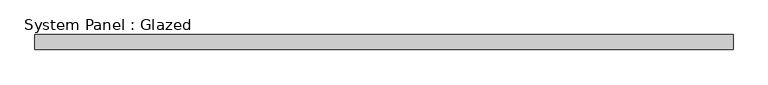
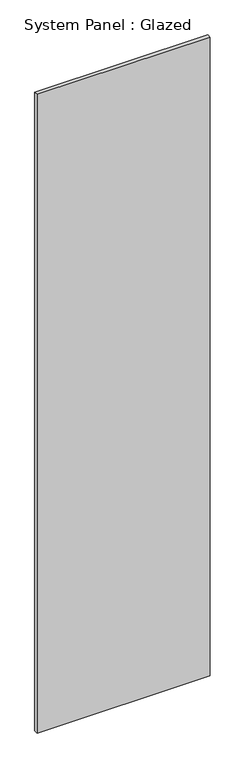
"""IFC4 building model written with IfcOpenShell, lengths in millimetres: plate geometry, System Panel : Glazed."""

import ifcopenshell
import ifcopenshell.guid

model = None  # the IFC model being written
_history = None  # IfcOwnerHistory: only IFC2X3 demands one
_inside = {}  # id of a spatial element -> (the spatial element, [elements in it])
_under = {}  # id of a project, library or spatial element -> (it, [spatial elements below it])
_declared = {}  # id of a project -> (the project, [libraries it declares])
_typed = {}  # id of a type object -> (the type object, [elements of that type])
_made_of = {}  # id of a material, layer set ... -> (it, [elements and type objects made of it])


def new_model(schema):
    """Start an empty IFC model of exactly this schema.

    Asked for "IFC4X3", IfcOpenShell would pick the latest addendum, in which some entities
    have other attributes; the version numbers below select the first issue.
    IFC2X3 requires an IfcOwnerHistory on every rooted entity: one is made here for all.
    """
    global model, _history
    if schema == "IFC4X3":
        model = ifcopenshell.file(schema_version=(4, 3, 0, 0))
    else:
        model = ifcopenshell.file(schema=schema)
    _inside.clear()
    _under.clear()
    _declared.clear()
    _typed.clear()
    _made_of.clear()
    _history = None
    if model.schema == "IFC2X3":
        org = make("IfcOrganization", Name="unknown")
        user = make(
            "IfcPersonAndOrganization",
            ThePerson=make("IfcPerson", FamilyName="unknown"),
            TheOrganization=org,
        )
        app = make(
            "IfcApplication",
            ApplicationDeveloper=org,
            Version="unknown",
            ApplicationFullName="unknown",
            ApplicationIdentifier="unknown",
        )
        _history = make(
            "IfcOwnerHistory",
            OwningUser=user,
            OwningApplication=app,
            ChangeAction="ADDED",
            CreationDate=0,
        )
    return model


def make(cls, **values):
    """One entity of the class cls with the attributes given. An attribute that is None is left unset."""
    return model.create_entity(
        cls, **{name: value for name, value in values.items() if value is not None}
    )


def rooted(cls, **values):
    """An entity with a GlobalId (a new one), such as an element, a storey or a relation."""
    return make(cls, GlobalId=ifcopenshell.guid.new(), OwnerHistory=_history, **values)


def si_unit(unit_type, name, prefix=None):
    """IfcSIUnit, for example si_unit("LENGTHUNIT", "METRE", prefix="MILLI")."""
    return make("IfcSIUnit", UnitType=unit_type, Prefix=prefix, Name=name)


def assignment(units):
    """IfcUnitAssignment: the units of a project."""
    return None if units is None else make("IfcUnitAssignment", Units=units)


def point(xyz):
    """IfcCartesianPoint."""
    return None if xyz is None else make("IfcCartesianPoint", Coordinates=xyz)


def direction(xyz):
    """IfcDirection."""
    return None if xyz is None else make("IfcDirection", DirectionRatios=xyz)


def frame(location, z_axis=None, x_axis=None):
    """IfcAxis2Placement3D, a coordinate frame: its origin and axes. An axis left out is left unset."""
    return make(
        "IfcAxis2Placement3D",
        Location=point(location),
        Axis=direction(z_axis),
        RefDirection=direction(x_axis),
    )


def origin():
    """The frame at (0, 0, 0) with its axes left unset."""
    return frame((0.0, 0.0, 0.0))


def origin_with_axes():
    """The frame at (0, 0, 0) with the z axis (0, 0, 1) and the x axis (1, 0, 0) written out."""
    return frame((0.0, 0.0, 0.0), z_axis=(0.0, 0.0, 1.0), x_axis=(1.0, 0.0, 0.0))


def place(relative_to, where):
    """IfcLocalPlacement: puts the frame where relative to a parent placement (None: the world)."""
    return make(
        "IfcLocalPlacement", PlacementRelTo=relative_to, RelativePlacement=where
    )


def context(
    kind, dimensions, precision=None, world=None, true_north=None, identifier=None
):
    """IfcGeometricRepresentationContext, for example the 3D "Model" context."""
    return make(
        "IfcGeometricRepresentationContext",
        ContextIdentifier=identifier,
        ContextType=kind,
        CoordinateSpaceDimension=dimensions,
        Precision=precision,
        WorldCoordinateSystem=world,
        TrueNorth=true_north,
    )


def project(units=None, contexts=None):
    """IfcProject with its units and contexts."""
    return rooted(
        "IfcProject",
        Name="project",
        RepresentationContexts=contexts,
        UnitsInContext=assignment(units),
    )


def spatial(cls, under=None, at=None, **own):
    """A site, building, storey or space (cls), placed at a placement, below another one or the project."""
    s = rooted(cls, ObjectPlacement=at, **own)
    if under is not None:
        _under.setdefault(under.id(), (under, []))[1].append(s)
    return s


def polyline(points):
    """IfcPolyline through the points."""
    return make("IfcPolyline", Points=[point(p) for p in points])


def outline(outer, holes=None, kind="AREA"):
    """IfcArbitraryClosedProfileDef: a profile drawn as a closed curve; with holes, ...WithVoids."""
    if holes is None:
        return make("IfcArbitraryClosedProfileDef", ProfileType=kind, OuterCurve=outer)
    return make(
        "IfcArbitraryProfileDefWithVoids",
        ProfileType=kind,
        OuterCurve=outer,
        InnerCurves=holes,
    )


def extrude(swept, where, along, depth):
    """IfcExtrudedAreaSolid: the profile swept, set in the frame where, extruded along a direction by depth."""
    return make(
        "IfcExtrudedAreaSolid",
        SweptArea=swept,
        Position=where,
        ExtrudedDirection=direction(along),
        Depth=depth,
    )


def shape(context_of_items, identifier, shape_type, items):
    """IfcShapeRepresentation: the items that make up one representation, for example the "Body"."""
    return make(
        "IfcShapeRepresentation",
        ContextOfItems=context_of_items,
        RepresentationIdentifier=identifier,
        RepresentationType=shape_type,
        Items=items,
    )


def source(mapping_origin, context_of_items, identifier, shape_type, items):
    """IfcRepresentationMap: a shape defined once, which mapped items show again and again."""
    return make(
        "IfcRepresentationMap",
        MappingOrigin=mapping_origin,
        MappedRepresentation=shape(context_of_items, identifier, shape_type, items),
    )


def transform(
    local_origin,
    x_axis=None,
    y_axis=None,
    z_axis=None,
    scale=None,
    scale2=None,
    scale3=None,
    uniform=True,
):
    """IfcCartesianTransformationOperator3D, or its non-uniform kind. x_axis, y_axis, z_axis: its Axis1, 2, 3."""
    if uniform:
        return make(
            "IfcCartesianTransformationOperator3D",
            Axis1=direction(x_axis),
            Axis2=direction(y_axis),
            LocalOrigin=point(local_origin),
            Scale=scale,
            Axis3=direction(z_axis),
        )
    return make(
        "IfcCartesianTransformationOperator3DnonUniform",
        Axis1=direction(x_axis),
        Axis2=direction(y_axis),
        LocalOrigin=point(local_origin),
        Scale=scale,
        Axis3=direction(z_axis),
        Scale2=scale2,
        Scale3=scale3,
    )


def mapped(mapping_source, mapping_target):
    """IfcMappedItem: shows the shape of a source again, moved by a transform."""
    return make(
        "IfcMappedItem", MappingSource=mapping_source, MappingTarget=mapping_target
    )


def made_of(thing, what):
    """Note that an element or type object is made of a material, layer set ...; save() writes the relation."""
    if what is not None:
        _made_of.setdefault(what.id(), (what, []))[1].append(thing)
    return thing


def element(
    cls,
    number,
    at=None,
    inside=None,
    cuts=None,
    type_object=None,
    material=None,
    context=None,
    identifier="Body",
    shape_type=None,
    held_by="IfcProductDefinitionShape",
    body=None,
    shapes=None,
    **own,
):
    """One element of the class cls, such as IfcWall. Its Tag is "e" and its number.

    at: its placement. inside: the storey or other place that contains it. cuts: it is an
    opening in that element (IfcRelVoidsElement). A single representation is given by context,
    identifier, shape_type and body (its items); several are given by shapes. held_by: the class
    of the entity that holds the representations. save() writes the other relations.
    """
    e = rooted(cls, Tag="e%d" % number, ObjectPlacement=at, **own)
    if body is not None:
        shapes = [shape(context, identifier, shape_type, body)]
    if shapes is not None:
        e.Representation = make(held_by, Representations=shapes)
    if inside is not None:
        _inside.setdefault(inside.id(), (inside, []))[1].append(e)
    if cuts is not None:
        rooted(
            "IfcRelVoidsElement", RelatingBuildingElement=cuts, RelatedOpeningElement=e
        )
    if type_object is not None:
        _typed.setdefault(type_object.id(), (type_object, []))[1].append(e)
    return made_of(e, material)


def aggregate(whole, parts):
    """IfcRelAggregates: a whole, such as a stair, and the parts it consists of."""
    return rooted("IfcRelAggregates", RelatingObject=whole, RelatedObjects=parts)


def save(model, path):
    """Write the relations noted so far, then the file.

    IfcRelAggregates (storeys below a building ...), IfcRelContainedInSpatialStructure (elements
    in a storey), IfcRelDefinesByType, IfcRelAssociatesMaterial and IfcRelDeclares: one each for
    every whole, place, type object, material and project.
    """
    for whole, parts in _under.values():
        aggregate(whole, parts)
    for where, things in _inside.values():
        rooted(
            "IfcRelContainedInSpatialStructure",
            RelatedElements=things,
            RelatingStructure=where,
        )
    for kind, things in _typed.values():
        rooted("IfcRelDefinesByType", RelatedObjects=things, RelatingType=kind)
    for what, things in _made_of.values():
        rooted("IfcRelAssociatesMaterial", RelatedObjects=things, RelatingMaterial=what)
    for by, libraries in _declared.values():
        rooted("IfcRelDeclares", RelatingContext=by, RelatedDefinitions=libraries)
    model.write(path)


def system_panel_glazed_908aa4c7(model_context):
    return source(origin(), model_context, "Body", "SweptSolid", [
        extrude(outline(polyline([(593.725, 19.05), (-593.725, 19.05), (-593.725, 44.45), (593.725, 44.45), (593.725, 19.05)])), origin_with_axes(), (0.0, 0.0, 1.0), 4629.15),
    ])


if __name__ == "__main__":
    model = new_model("IFC4")
    model_context = context("Model", 3, world=origin())
    ifc_project = project(units=[si_unit("LENGTHUNIT", "METRE", prefix="MILLI")], contexts=[model_context])
    site = spatial("IfcSite", under=ifc_project)
    building = spatial("IfcBuilding", under=site)
    placement = place(None, origin())
    system_panel_glazed_shape = system_panel_glazed_908aa4c7(model_context)
    element("IfcPlate", 1, ObjectType="System Panel : Glazed", at=placement, inside=building, context=model_context, shape_type="MappedRepresentation", body=[
        mapped(system_panel_glazed_shape, transform((0.0, 0.0, 0.0), x_axis=(1.0, 0.0, 0.0), y_axis=(0.0, 1.0, 0.0), z_axis=(0.0, 0.0, 1.0))),
    ])
    save(model, "model.ifc")

# Revit data of these elements
# Type "System Panel : Glazed"
#   Construction Type Id = "GSP4R"
#   Analytic Construction = "1/8 in Pilkington single glazing"
#   Visual Light Transmittance = 0.9
#   Solar Heat Gain Coefficient = 0.86
#   Heat Transfer Coefficient (U) = 1.18115 BTU/(h·ft²·°F)
#   Define Thermal Properties by = 1
# Element 1 (IfcPlate, "System Panel : Glazed")
#   Materials on its faces: "Glass"
# Materials
#   "Glass": class "Glass", colour RGB 0 128 192, transparency 0.75, Description = "Soda Lime Glass", Cost = 0
